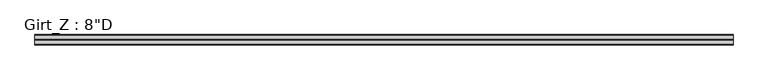
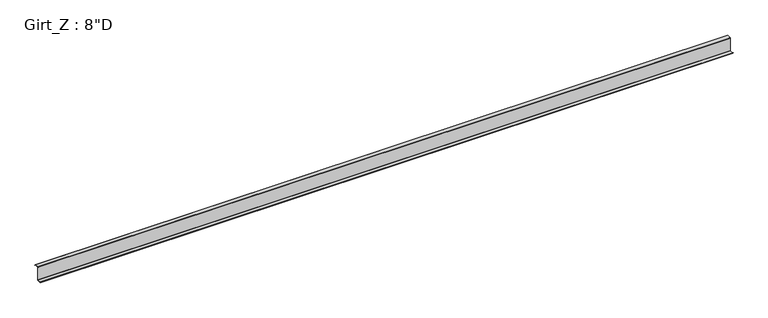
"""IFC4 building model written with IfcOpenShell, lengths in millimetres: beam geometry."""

from ifc_helpers import new_model, si_unit, point, frame, frame_2d, origin, place, context, project, spatial, polyline, circle_curve, trimmed, segment, composite_curve, outline, extrude, source, transform, mapped, element, save


def beam_f7fad3c8(model_context):
    return source(origin(), model_context, "Body", "SweptSolid", [
        extrude(outline(composite_curve([segment(polyline([(63.5, 101.6), (75.745104, 87.0068534), (73.6169367, 85.221109), (62.204539, 98.821875), (3.3005807, 98.821875)]), True, "CONTINUOUS"), segment(trimmed(circle_curve(frame_2d((3.3741066, 96.8381931)), 1.9850441), [point((3.3005807, 98.821875))], [point((1.3890625, 96.8381931))], True, "CARTESIAN"), True, "CONTINUOUS"), segment(polyline([(1.3890625, 96.8381931), (1.3890625, -96.8375)]), True, "CONTINUOUS"), segment(trimmed(circle_curve(frame_2d((-3.3734375, -96.8375)), 4.7625), [point((1.3890625, -96.8375))], [point((-3.3734375, -101.6))], False, "CARTESIAN"), True, "CONTINUOUS"), segment(polyline([(-3.3734375, -101.6), (-63.5, -101.6), (-75.745104, -87.0068534), (-73.6169367, -85.221109), (-62.204539, -98.821875), (-3.2694106, -98.821875)]), True, "CONTINUOUS"), segment(trimmed(circle_curve(frame_2d((-3.3748024, -96.8389339)), 1.9857399), [point((-3.2694106, -98.821875))], [point((-1.3890625, -96.8389339))], True, "CARTESIAN"), True, "CONTINUOUS"), segment(polyline([(-1.3890625, -96.8389339), (-1.3890625, 96.8375)]), True, "CONTINUOUS"), segment(trimmed(circle_curve(frame_2d((3.3734375, 96.8375)), 4.7625), [point((-1.3890625, 96.8375))], [point((3.3734375, 101.6))], False, "CARTESIAN"), True, "CONTINUOUS"), segment(polyline([(3.3734375, 101.6), (63.5, 101.6)]), True, "CONTINUOUS")], self_intersect=False)), frame((-5139.310137, 0.0, 0.0), z_axis=(1.0, 0.0, 0.0), x_axis=(0.0, 1.0, 0.0)), (0.0, 0.0, 1.0), 10267.1311828),
    ])


if __name__ == "__main__":
    model = new_model("IFC4")
    model_context = context("Model", 3, world=origin())
    ifc_project = project(units=[si_unit("LENGTHUNIT", "METRE", prefix="MILLI")], contexts=[model_context])
    site = spatial("IfcSite", under=ifc_project)
    building = spatial("IfcBuilding", under=site)
    placement = place(None, origin())
    beam_shape = beam_f7fad3c8(model_context)
    element("IfcBeam", 1, ObjectType="Girt_Z : 8\"D", at=placement, inside=building, context=model_context, shape_type="MappedRepresentation", body=[
        mapped(beam_shape, transform((0.0, 0.0, 0.0), x_axis=(1.0, 0.0, 0.0), y_axis=(0.0, 1.0, 0.0), z_axis=(0.0, 0.0, 1.0))),
    ])
    save(model, "model.ifc")

# Revit data of these elements
# Type "Girt_Z : 8\"D"
#   Web_Thickness = 0' - 0 7/64"
#   Length [instance default] = 10' - 0"
#   Leg_1 = 0' - 2 1/2"
#   Height = 0' - 8"
#   Structural Material [instance default] = none
# Element 1 (IfcBeam, "Girt_Z : 8\"D")
#   Structural Material = Steel
#   Materials on its faces: "Steel"
# Materials
#   "Steel": class "Metal", colour RGB 118 118 114, transparency 0, Description = "Steel, mill finish", Cost = 0
